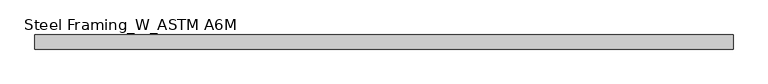
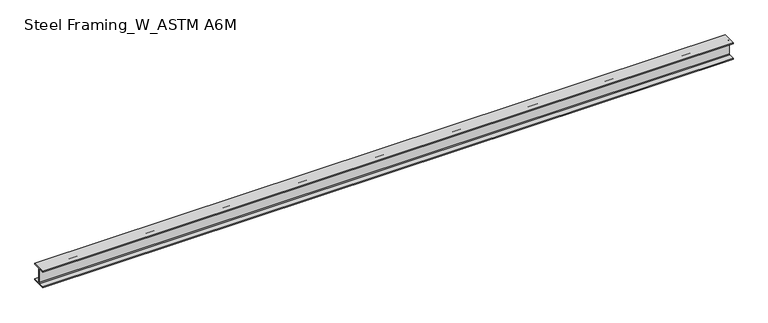
"""IFC4 building model written with IfcOpenShell, lengths in millimetres: beam geometry, Steel Framing_W_ASTM A6M : H_SB_AR_S02_W250x49.1_RB3."""

import ifcopenshell
import ifcopenshell.guid

model = None  # the IFC model being written
_history = None  # IfcOwnerHistory: only IFC2X3 demands one
_inside = {}  # id of a spatial element -> (the spatial element, [elements in it])
_under = {}  # id of a project, library or spatial element -> (it, [spatial elements below it])
_declared = {}  # id of a project -> (the project, [libraries it declares])
_typed = {}  # id of a type object -> (the type object, [elements of that type])
_made_of = {}  # id of a material, layer set ... -> (it, [elements and type objects made of it])


def new_model(schema):
    """Start an empty IFC model of exactly this schema.

    Asked for "IFC4X3", IfcOpenShell would pick the latest addendum, in which some entities
    have other attributes; the version numbers below select the first issue.
    IFC2X3 requires an IfcOwnerHistory on every rooted entity: one is made here for all.
    """
    global model, _history
    if schema == "IFC4X3":
        model = ifcopenshell.file(schema_version=(4, 3, 0, 0))
    else:
        model = ifcopenshell.file(schema=schema)
    _inside.clear()
    _under.clear()
    _declared.clear()
    _typed.clear()
    _made_of.clear()
    _history = None
    if model.schema == "IFC2X3":
        org = make("IfcOrganization", Name="unknown")
        user = make(
            "IfcPersonAndOrganization",
            ThePerson=make("IfcPerson", FamilyName="unknown"),
            TheOrganization=org,
        )
        app = make(
            "IfcApplication",
            ApplicationDeveloper=org,
            Version="unknown",
            ApplicationFullName="unknown",
            ApplicationIdentifier="unknown",
        )
        _history = make(
            "IfcOwnerHistory",
            OwningUser=user,
            OwningApplication=app,
            ChangeAction="ADDED",
            CreationDate=0,
        )
    return model


def make(cls, **values):
    """One entity of the class cls with the attributes given. An attribute that is None is left unset."""
    return model.create_entity(
        cls, **{name: value for name, value in values.items() if value is not None}
    )


def rooted(cls, **values):
    """An entity with a GlobalId (a new one), such as an element, a storey or a relation."""
    return make(cls, GlobalId=ifcopenshell.guid.new(), OwnerHistory=_history, **values)


def si_unit(unit_type, name, prefix=None):
    """IfcSIUnit, for example si_unit("LENGTHUNIT", "METRE", prefix="MILLI")."""
    return make("IfcSIUnit", UnitType=unit_type, Prefix=prefix, Name=name)


def assignment(units):
    """IfcUnitAssignment: the units of a project."""
    return None if units is None else make("IfcUnitAssignment", Units=units)


def point(xyz):
    """IfcCartesianPoint."""
    return None if xyz is None else make("IfcCartesianPoint", Coordinates=xyz)


def direction(xyz):
    """IfcDirection."""
    return None if xyz is None else make("IfcDirection", DirectionRatios=xyz)


def frame(location, z_axis=None, x_axis=None):
    """IfcAxis2Placement3D, a coordinate frame: its origin and axes. An axis left out is left unset."""
    return make(
        "IfcAxis2Placement3D",
        Location=point(location),
        Axis=direction(z_axis),
        RefDirection=direction(x_axis),
    )


def frame_2d(location, x_axis=None):
    """IfcAxis2Placement2D, a coordinate frame in the plane: its origin and x axis."""
    return make(
        "IfcAxis2Placement2D", Location=point(location), RefDirection=direction(x_axis)
    )


def origin():
    """The frame at (0, 0, 0) with its axes left unset."""
    return frame((0.0, 0.0, 0.0))


def place(relative_to, where):
    """IfcLocalPlacement: puts the frame where relative to a parent placement (None: the world)."""
    return make(
        "IfcLocalPlacement", PlacementRelTo=relative_to, RelativePlacement=where
    )


def context(
    kind, dimensions, precision=None, world=None, true_north=None, identifier=None
):
    """IfcGeometricRepresentationContext, for example the 3D "Model" context."""
    return make(
        "IfcGeometricRepresentationContext",
        ContextIdentifier=identifier,
        ContextType=kind,
        CoordinateSpaceDimension=dimensions,
        Precision=precision,
        WorldCoordinateSystem=world,
        TrueNorth=true_north,
    )


def project(units=None, contexts=None):
    """IfcProject with its units and contexts."""
    return rooted(
        "IfcProject",
        Name="project",
        RepresentationContexts=contexts,
        UnitsInContext=assignment(units),
    )


def spatial(cls, under=None, at=None, **own):
    """A site, building, storey or space (cls), placed at a placement, below another one or the project."""
    s = rooted(cls, ObjectPlacement=at, **own)
    if under is not None:
        _under.setdefault(under.id(), (under, []))[1].append(s)
    return s


def polyline(points):
    """IfcPolyline through the points."""
    return make("IfcPolyline", Points=[point(p) for p in points])


def circle_curve(where, radius):
    """IfcCircle in the frame where."""
    return make("IfcCircle", Position=where, Radius=radius)


def trimmed(basis, trim1, trim2, sense, master):
    """IfcTrimmedCurve: the piece of a basis curve between two trims."""
    return make(
        "IfcTrimmedCurve",
        BasisCurve=basis,
        Trim1=trim1,
        Trim2=trim2,
        SenseAgreement=sense,
        MasterRepresentation=master,
    )


def segment(curve, same_sense, transition):
    """IfcCompositeCurveSegment."""
    return make(
        "IfcCompositeCurveSegment",
        Transition=transition,
        SameSense=same_sense,
        ParentCurve=curve,
    )


def composite_curve(segments, self_intersect=None):
    """IfcCompositeCurve: segments joined end to end."""
    return make("IfcCompositeCurve", Segments=segments, SelfIntersect=self_intersect)


def outline(outer, holes=None, kind="AREA"):
    """IfcArbitraryClosedProfileDef: a profile drawn as a closed curve; with holes, ...WithVoids."""
    if holes is None:
        return make("IfcArbitraryClosedProfileDef", ProfileType=kind, OuterCurve=outer)
    return make(
        "IfcArbitraryProfileDefWithVoids",
        ProfileType=kind,
        OuterCurve=outer,
        InnerCurves=holes,
    )


def extrude(swept, where, along, depth):
    """IfcExtrudedAreaSolid: the profile swept, set in the frame where, extruded along a direction by depth."""
    return make(
        "IfcExtrudedAreaSolid",
        SweptArea=swept,
        Position=where,
        ExtrudedDirection=direction(along),
        Depth=depth,
    )


def shape(context_of_items, identifier, shape_type, items):
    """IfcShapeRepresentation: the items that make up one representation, for example the "Body"."""
    return make(
        "IfcShapeRepresentation",
        ContextOfItems=context_of_items,
        RepresentationIdentifier=identifier,
        RepresentationType=shape_type,
        Items=items,
    )


def source(mapping_origin, context_of_items, identifier, shape_type, items):
    """IfcRepresentationMap: a shape defined once, which mapped items show again and again."""
    return make(
        "IfcRepresentationMap",
        MappingOrigin=mapping_origin,
        MappedRepresentation=shape(context_of_items, identifier, shape_type, items),
    )


def transform(
    local_origin,
    x_axis=None,
    y_axis=None,
    z_axis=None,
    scale=None,
    scale2=None,
    scale3=None,
    uniform=True,
):
    """IfcCartesianTransformationOperator3D, or its non-uniform kind. x_axis, y_axis, z_axis: its Axis1, 2, 3."""
    if uniform:
        return make(
            "IfcCartesianTransformationOperator3D",
            Axis1=direction(x_axis),
            Axis2=direction(y_axis),
            LocalOrigin=point(local_origin),
            Scale=scale,
            Axis3=direction(z_axis),
        )
    return make(
        "IfcCartesianTransformationOperator3DnonUniform",
        Axis1=direction(x_axis),
        Axis2=direction(y_axis),
        LocalOrigin=point(local_origin),
        Scale=scale,
        Axis3=direction(z_axis),
        Scale2=scale2,
        Scale3=scale3,
    )


def mapped(mapping_source, mapping_target):
    """IfcMappedItem: shows the shape of a source again, moved by a transform."""
    return make(
        "IfcMappedItem", MappingSource=mapping_source, MappingTarget=mapping_target
    )


def made_of(thing, what):
    """Note that an element or type object is made of a material, layer set ...; save() writes the relation."""
    if what is not None:
        _made_of.setdefault(what.id(), (what, []))[1].append(thing)
    return thing


def element(
    cls,
    number,
    at=None,
    inside=None,
    cuts=None,
    type_object=None,
    material=None,
    context=None,
    identifier="Body",
    shape_type=None,
    held_by="IfcProductDefinitionShape",
    body=None,
    shapes=None,
    **own,
):
    """One element of the class cls, such as IfcWall. Its Tag is "e" and its number.

    at: its placement. inside: the storey or other place that contains it. cuts: it is an
    opening in that element (IfcRelVoidsElement). A single representation is given by context,
    identifier, shape_type and body (its items); several are given by shapes. held_by: the class
    of the entity that holds the representations. save() writes the other relations.
    """
    e = rooted(cls, Tag="e%d" % number, ObjectPlacement=at, **own)
    if body is not None:
        shapes = [shape(context, identifier, shape_type, body)]
    if shapes is not None:
        e.Representation = make(held_by, Representations=shapes)
    if inside is not None:
        _inside.setdefault(inside.id(), (inside, []))[1].append(e)
    if cuts is not None:
        rooted(
            "IfcRelVoidsElement", RelatingBuildingElement=cuts, RelatedOpeningElement=e
        )
    if type_object is not None:
        _typed.setdefault(type_object.id(), (type_object, []))[1].append(e)
    return made_of(e, material)


def aggregate(whole, parts):
    """IfcRelAggregates: a whole, such as a stair, and the parts it consists of."""
    return rooted("IfcRelAggregates", RelatingObject=whole, RelatedObjects=parts)


def save(model, path):
    """Write the relations noted so far, then the file.

    IfcRelAggregates (storeys below a building ...), IfcRelContainedInSpatialStructure (elements
    in a storey), IfcRelDefinesByType, IfcRelAssociatesMaterial and IfcRelDeclares: one each for
    every whole, place, type object, material and project.
    """
    for whole, parts in _under.values():
        aggregate(whole, parts)
    for where, things in _inside.values():
        rooted(
            "IfcRelContainedInSpatialStructure",
            RelatedElements=things,
            RelatingStructure=where,
        )
    for kind, things in _typed.values():
        rooted("IfcRelDefinesByType", RelatedObjects=things, RelatingType=kind)
    for what, things in _made_of.values():
        rooted("IfcRelAssociatesMaterial", RelatedObjects=things, RelatingMaterial=what)
    for by, libraries in _declared.values():
        rooted("IfcRelDeclares", RelatingContext=by, RelatedDefinitions=libraries)
    model.write(path)


def steel_framing_w_astm_a6m_504daf18(model_context):
    return source(origin(), model_context, "Body", "SweptSolid", [
        extrude(outline(composite_curve([segment(polyline([(101.0, -112.5), (101.0, -123.5), (-101.0, -123.5), (-101.0, -112.5), (-16.385, -112.5)]), True, "CONTINUOUS"), segment(trimmed(circle_curve(frame_2d((-16.385, -99.8)), 12.7), [point((-16.385, -112.5))], [point((-3.685, -99.8))], True, "CARTESIAN"), True, "CONTINUOUS"), segment(polyline([(-3.685, -99.8), (-3.685, 99.8)]), True, "CONTINUOUS"), segment(trimmed(circle_curve(frame_2d((-16.385, 99.8)), 12.7), [point((-3.685, 99.8))], [point((-16.385, 112.5))], True, "CARTESIAN"), True, "CONTINUOUS"), segment(polyline([(-16.385, 112.5), (-101.0, 112.5), (-101.0, 123.5), (101.0, 123.5), (101.0, 112.5), (16.385, 112.5)]), True, "CONTINUOUS"), segment(trimmed(circle_curve(frame_2d((16.385, 99.8)), 12.7), [point((16.385, 112.5))], [point((3.685, 99.8))], True, "CARTESIAN"), True, "CONTINUOUS"), segment(polyline([(3.685, 99.8), (3.685, -99.8)]), True, "CONTINUOUS"), segment(trimmed(circle_curve(frame_2d((16.385, -99.8)), 12.7), [point((3.685, -99.8))], [point((16.385, -112.5))], True, "CARTESIAN"), True, "CONTINUOUS"), segment(polyline([(16.385, -112.5), (101.0, -112.5)]), True, "CONTINUOUS")], self_intersect=False)), frame((-5000.0, 0.0, 0.0), z_axis=(1.0, 0.0, 0.0), x_axis=(0.0, 1.0, 0.0)), (0.0, 0.0, 1.0), 9987.2),
    ])


if __name__ == "__main__":
    model = new_model("IFC4")
    model_context = context("Model", 3, world=origin())
    ifc_project = project(units=[si_unit("LENGTHUNIT", "METRE", prefix="MILLI")], contexts=[model_context])
    site = spatial("IfcSite", under=ifc_project)
    building = spatial("IfcBuilding", under=site)
    placement = place(None, origin())
    steel_framing_w_astm_a6m_shape = steel_framing_w_astm_a6m_504daf18(model_context)
    element("IfcBeam", 1, ObjectType="Steel Framing_W_ASTM A6M : H_SB_AR_S02_W250x49.1_RB3", at=placement, inside=building, context=model_context, shape_type="MappedRepresentation", body=[
        mapped(steel_framing_w_astm_a6m_shape, transform((0.0, 0.0, 0.0), x_axis=(1.0, 0.0, 0.0), y_axis=(0.0, 1.0, 0.0), z_axis=(0.0, 0.0, 1.0))),
    ])
    save(model, "model.ifc")

# Revit data of these elements
# Type "Steel Framing_W_ASTM A6M : H_SB_AR_S02_W250x49.1_RB3"
#   Section Name Key = "W10x33"
#   Width = 20.2 cm
#   Web Thickness = 0.737 cm
#   Web Fillet = 1.27 cm
#   Warping Constant = 212000.0 cm⁶
#   Torsional Moment of Inertia = 24.30 cm⁴
#   Section Area = 62.6 cm²
#   Plastic Modulus weak axis = 229.0 cm³
#   Plastic Modulus strong axis = 636.0 cm³
#   Perimeter = 1.27 m²/m
#   Nominal Weight = 49.10 kgf/m
#   Moment of Inertia weak axis = 1520.00 cm⁴
#   Moment of Inertia strong axis = 7120.00 cm⁴
#   Height = 24.7 cm
#   Flange Thickness = 1.1 cm
#   Elastic Modulus weak axis = 151.0 cm³
#   Elastic Modulus strong axis = 574.0 cm³
#   Centroid Vertical = 12.35 cm
#   Centroid Horizontal = 10.1 cm
#   Length [instance default] = 1500 mm
#   Structural Material [instance default] = Steel, 45-345
#   Bolt Spacing = 0
#   Assembly Code = ""
# Element 1 (IfcBeam, "Steel Framing_W_ASTM A6M : H_SB_AR_S02_W250x49.1_RB3")
#   Materials on its faces: "Steel, 45-345"
# Materials
#   "Steel, 45-345": class "Metal", colour RGB 189 187 185, transparency 0, Description = "Steel 345 MPa", Cost = 0
